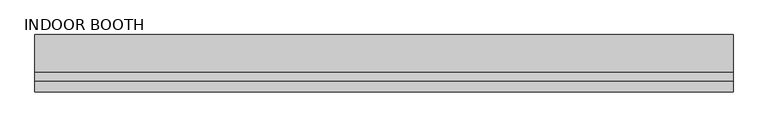
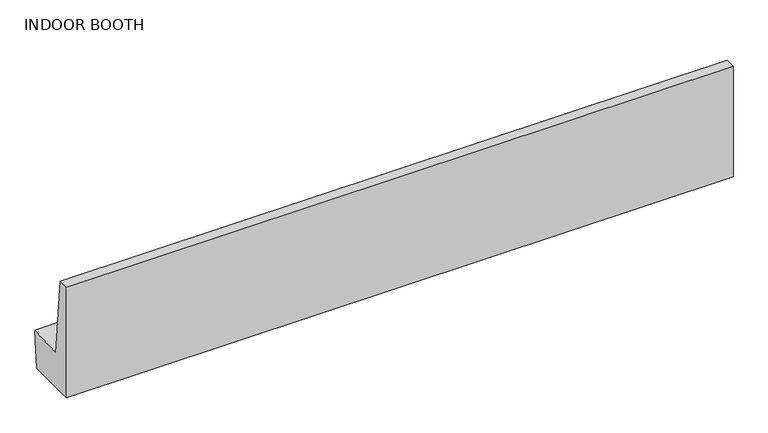
"""IFC4 building model written with IfcOpenShell, lengths in millimetres: furniture geometry, OD_CW_Booth : INDOOR BOOTH."""

from ifc_helpers import new_model, si_unit, frame, origin, place, context, project, spatial, polyline, outline, extrude, source, transform, mapped, element, save


def indoor_booth_16a05349(model_context):
    return source(origin(), model_context, "Body", "SweptSolid", [
        extrude(outline(polyline([(-609.6, 1397.0), (-484.4524721, 1397.0), (-382.9385128, 431.1591941), (43.0849153, 453.4861359), (3.4100193, 0.0), (-609.6, 0.0), (-609.6, 1397.0)])), frame((18.7377049, 0.0, 0.0), z_axis=(1.0, 0.0, 0.0), x_axis=(0.0, 1.0, 0.0)), (0.0, 0.0, 1.0), 7958.479089),
    ])


if __name__ == "__main__":
    model = new_model("IFC4")
    model_context = context("Model", 3, world=origin())
    ifc_project = project(units=[si_unit("LENGTHUNIT", "METRE", prefix="MILLI")], contexts=[model_context])
    site = spatial("IfcSite", under=ifc_project)
    building = spatial("IfcBuilding", under=site)
    placement = place(None, origin())
    indoor_booth_shape = indoor_booth_16a05349(model_context)
    element("IfcFurniture", 1, ObjectType="OD_CW_Booth : INDOOR BOOTH", at=placement, inside=building, context=model_context, shape_type="MappedRepresentation", body=[
        mapped(indoor_booth_shape, transform((0.0, 0.0, 0.0), x_axis=(1.0, 0.0, 0.0), y_axis=(0.0, 1.0, 0.0), z_axis=(0.0, 0.0, 1.0))),
    ])
    save(model, "model.ifc")

# Revit data of these elements
# Type "OD_CW_Booth : INDOOR BOOTH"
#   Type Mark = "TYPE-INDOOR"
#   Width = 4' - 0"
#   OD_CW_Width [instance default] = 2' - 10"
#   OD_CW_Length [instance default] = 26' - 1 83/256"
#   OD_CW_Height [instance default] = 2' - 3"
#   Height = 3' - 0"
#   Depth = 2' - 0"
#   Seating Count [instance default] = 10
#   Seating Count [instance default] = 10
#   OD_CW_Material_Front Panel [instance default] = none
#   OD_CW_Material_Body [instance default] = none
# Element 1 (IfcFurniture, "OD_CW_Booth : INDOOR BOOTH")
#   OD_CW_Length = 26' - 1.32595"
#   OD_CW_Material_Body = Sals Wood
#   Materials on its faces: "Sals Wood"
# Materials
#   "Sals Wood": class "Wood", colour RGB 198 202 183, transparency 0, Description = "Generic wood", Cost = 0
